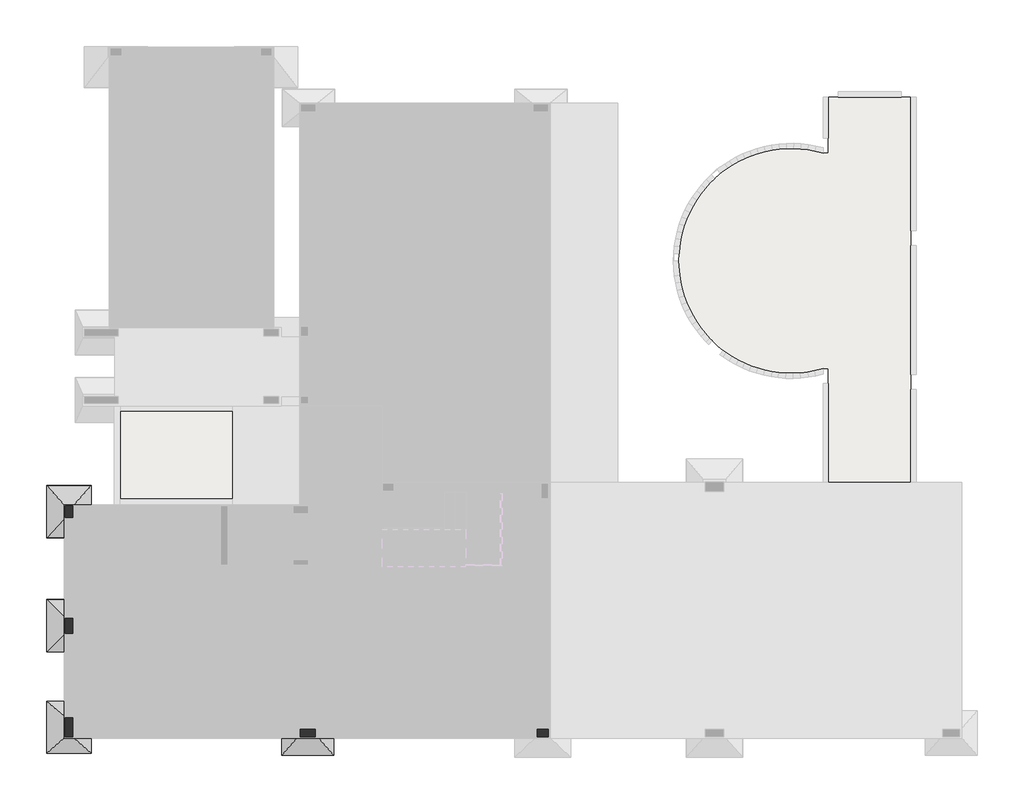
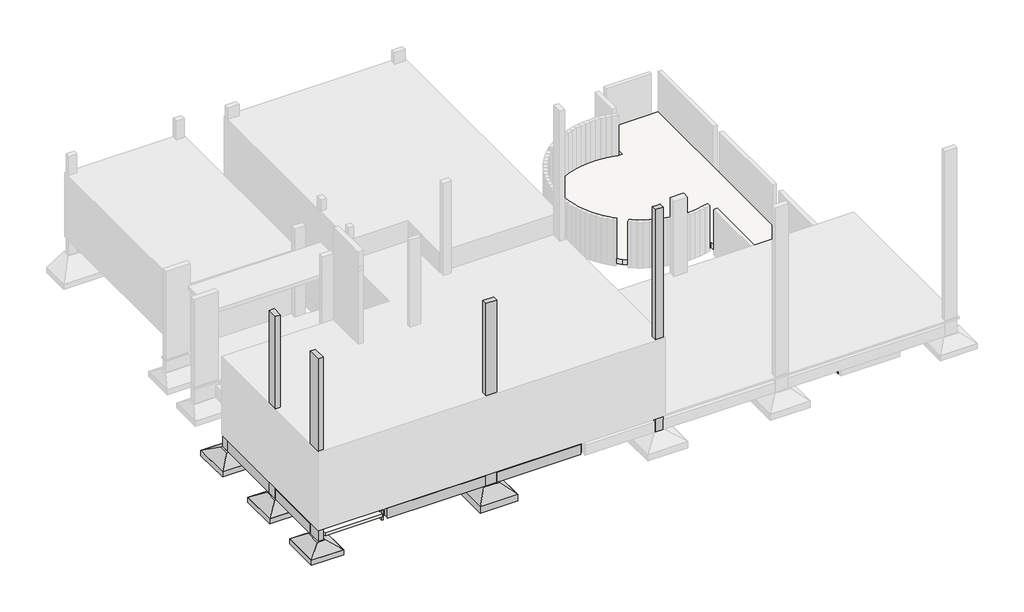
# One storey, part 1 of 4: 11 beams, 5 columns, 4 fasteners, 3 slabs.
"""IFC4 building model written with IfcOpenShell, lengths in millimetres."""

import ifcopenshell
import ifcopenshell.guid

model = None  # the IFC model being written
_history = None  # IfcOwnerHistory: only IFC2X3 demands one
_inside = {}  # id of a spatial element -> (the spatial element, [elements in it])
_under = {}  # id of a project, library or spatial element -> (it, [spatial elements below it])
_declared = {}  # id of a project -> (the project, [libraries it declares])
_typed = {}  # id of a type object -> (the type object, [elements of that type])
_made_of = {}  # id of a material, layer set ... -> (it, [elements and type objects made of it])


def new_model(schema):
    """Start an empty IFC model of exactly this schema.

    Asked for "IFC4X3", IfcOpenShell would pick the latest addendum, in which some entities
    have other attributes; the version numbers below select the first issue.
    IFC2X3 requires an IfcOwnerHistory on every rooted entity: one is made here for all.
    """
    global model, _history
    if schema == "IFC4X3":
        model = ifcopenshell.file(schema_version=(4, 3, 0, 0))
    else:
        model = ifcopenshell.file(schema=schema)
    _inside.clear()
    _under.clear()
    _declared.clear()
    _typed.clear()
    _made_of.clear()
    _history = None
    if model.schema == "IFC2X3":
        org = make("IfcOrganization", Name="unknown")
        user = make(
            "IfcPersonAndOrganization",
            ThePerson=make("IfcPerson", FamilyName="unknown"),
            TheOrganization=org,
        )
        app = make(
            "IfcApplication",
            ApplicationDeveloper=org,
            Version="unknown",
            ApplicationFullName="unknown",
            ApplicationIdentifier="unknown",
        )
        _history = make(
            "IfcOwnerHistory",
            OwningUser=user,
            OwningApplication=app,
            ChangeAction="ADDED",
            CreationDate=0,
        )
    return model


def make(cls, **values):
    """One entity of the class cls with the attributes given. An attribute that is None is left unset."""
    return model.create_entity(
        cls, **{name: value for name, value in values.items() if value is not None}
    )


def rooted(cls, **values):
    """An entity with a GlobalId (a new one), such as an element, a storey or a relation."""
    return make(cls, GlobalId=ifcopenshell.guid.new(), OwnerHistory=_history, **values)


def si_unit(unit_type, name, prefix=None):
    """IfcSIUnit, for example si_unit("LENGTHUNIT", "METRE", prefix="MILLI")."""
    return make("IfcSIUnit", UnitType=unit_type, Prefix=prefix, Name=name)


def assignment(units):
    """IfcUnitAssignment: the units of a project."""
    return None if units is None else make("IfcUnitAssignment", Units=units)


def point(xyz):
    """IfcCartesianPoint."""
    return None if xyz is None else make("IfcCartesianPoint", Coordinates=xyz)


def direction(xyz):
    """IfcDirection."""
    return None if xyz is None else make("IfcDirection", DirectionRatios=xyz)


def frame(location, z_axis=None, x_axis=None):
    """IfcAxis2Placement3D, a coordinate frame: its origin and axes. An axis left out is left unset."""
    return make(
        "IfcAxis2Placement3D",
        Location=point(location),
        Axis=direction(z_axis),
        RefDirection=direction(x_axis),
    )


def frame_2d(location, x_axis=None):
    """IfcAxis2Placement2D, a coordinate frame in the plane: its origin and x axis."""
    return make(
        "IfcAxis2Placement2D", Location=point(location), RefDirection=direction(x_axis)
    )


def origin():
    """The frame at (0, 0, 0) with its axes left unset."""
    return frame((0.0, 0.0, 0.0))


def place(relative_to, where):
    """IfcLocalPlacement: puts the frame where relative to a parent placement (None: the world)."""
    return make(
        "IfcLocalPlacement", PlacementRelTo=relative_to, RelativePlacement=where
    )


def context(
    kind, dimensions, precision=None, world=None, true_north=None, identifier=None
):
    """IfcGeometricRepresentationContext, for example the 3D "Model" context."""
    return make(
        "IfcGeometricRepresentationContext",
        ContextIdentifier=identifier,
        ContextType=kind,
        CoordinateSpaceDimension=dimensions,
        Precision=precision,
        WorldCoordinateSystem=world,
        TrueNorth=true_north,
    )


def project(units=None, contexts=None):
    """IfcProject with its units and contexts."""
    return rooted(
        "IfcProject",
        Name="project",
        RepresentationContexts=contexts,
        UnitsInContext=assignment(units),
    )


def spatial(cls, under=None, at=None, **own):
    """A site, building, storey or space (cls), placed at a placement, below another one or the project."""
    s = rooted(cls, ObjectPlacement=at, **own)
    if under is not None:
        _under.setdefault(under.id(), (under, []))[1].append(s)
    return s


def polyline(points):
    """IfcPolyline through the points."""
    return make("IfcPolyline", Points=[point(p) for p in points])


def circle_curve(where, radius):
    """IfcCircle in the frame where."""
    return make("IfcCircle", Position=where, Radius=radius)


def trimmed(basis, trim1, trim2, sense, master):
    """IfcTrimmedCurve: the piece of a basis curve between two trims."""
    return make(
        "IfcTrimmedCurve",
        BasisCurve=basis,
        Trim1=trim1,
        Trim2=trim2,
        SenseAgreement=sense,
        MasterRepresentation=master,
    )


def segment(curve, same_sense, transition):
    """IfcCompositeCurveSegment."""
    return make(
        "IfcCompositeCurveSegment",
        Transition=transition,
        SameSense=same_sense,
        ParentCurve=curve,
    )


def composite_curve(segments, self_intersect=None):
    """IfcCompositeCurve: segments joined end to end."""
    return make("IfcCompositeCurve", Segments=segments, SelfIntersect=self_intersect)


def outline(outer, holes=None, kind="AREA"):
    """IfcArbitraryClosedProfileDef: a profile drawn as a closed curve; with holes, ...WithVoids."""
    if holes is None:
        return make("IfcArbitraryClosedProfileDef", ProfileType=kind, OuterCurve=outer)
    return make(
        "IfcArbitraryProfileDefWithVoids",
        ProfileType=kind,
        OuterCurve=outer,
        InnerCurves=holes,
    )


def extrude(swept, where, along, depth):
    """IfcExtrudedAreaSolid: the profile swept, set in the frame where, extruded along a direction by depth."""
    return make(
        "IfcExtrudedAreaSolid",
        SweptArea=swept,
        Position=where,
        ExtrudedDirection=direction(along),
        Depth=depth,
    )


def faces_of(points, faces, orient=None, outer=None):
    """IfcFace entities. A face is a list of loops; a loop is a list of indices into points, from 0.

    orient and outer hold one flag for each loop. By default every Orientation is true, the
    first loop of a face is its IfcFaceOuterBound and the others are IfcFaceBound.
    """
    made = []
    for i, loops in enumerate(faces):
        bounds = []
        for j, loop in enumerate(loops):
            is_outer = j == 0 if outer is None else outer[i][j]
            bounds.append(
                make(
                    "IfcFaceOuterBound" if is_outer else "IfcFaceBound",
                    Bound=make("IfcPolyLoop", Polygon=[points[k] for k in loop]),
                    Orientation=True if orient is None else orient[i][j],
                )
            )
        made.append(make("IfcFace", Bounds=bounds))
    return made


def faceted_brep(points, faces, orient=None, outer=None, voids=None):
    """IfcFacetedBrep: a solid bounded by flat faces; with voids (closed shells), ...WithVoids."""
    shared = [point(p) for p in points]
    hull = make("IfcClosedShell", CfsFaces=faces_of(shared, faces, orient, outer))
    if voids is None:
        return make("IfcFacetedBrep", Outer=hull)
    return make(
        "IfcFacetedBrepWithVoids",
        Outer=hull,
        Voids=[
            make(cls, CfsFaces=faces_of(shared, fs, o, b)) for cls, fs, o, b in voids
        ],
    )


def shape(context_of_items, identifier, shape_type, items):
    """IfcShapeRepresentation: the items that make up one representation, for example the "Body"."""
    return make(
        "IfcShapeRepresentation",
        ContextOfItems=context_of_items,
        RepresentationIdentifier=identifier,
        RepresentationType=shape_type,
        Items=items,
    )


def source(mapping_origin, context_of_items, identifier, shape_type, items):
    """IfcRepresentationMap: a shape defined once, which mapped items show again and again."""
    return make(
        "IfcRepresentationMap",
        MappingOrigin=mapping_origin,
        MappedRepresentation=shape(context_of_items, identifier, shape_type, items),
    )


def transform(
    local_origin,
    x_axis=None,
    y_axis=None,
    z_axis=None,
    scale=None,
    scale2=None,
    scale3=None,
    uniform=True,
):
    """IfcCartesianTransformationOperator3D, or its non-uniform kind. x_axis, y_axis, z_axis: its Axis1, 2, 3."""
    if uniform:
        return make(
            "IfcCartesianTransformationOperator3D",
            Axis1=direction(x_axis),
            Axis2=direction(y_axis),
            LocalOrigin=point(local_origin),
            Scale=scale,
            Axis3=direction(z_axis),
        )
    return make(
        "IfcCartesianTransformationOperator3DnonUniform",
        Axis1=direction(x_axis),
        Axis2=direction(y_axis),
        LocalOrigin=point(local_origin),
        Scale=scale,
        Axis3=direction(z_axis),
        Scale2=scale2,
        Scale3=scale3,
    )


def mapped(mapping_source, mapping_target):
    """IfcMappedItem: shows the shape of a source again, moved by a transform."""
    return make(
        "IfcMappedItem", MappingSource=mapping_source, MappingTarget=mapping_target
    )


def made_of(thing, what):
    """Note that an element or type object is made of a material, layer set ...; save() writes the relation."""
    if what is not None:
        _made_of.setdefault(what.id(), (what, []))[1].append(thing)
    return thing


def element(
    cls,
    number,
    at=None,
    inside=None,
    cuts=None,
    type_object=None,
    material=None,
    context=None,
    identifier="Body",
    shape_type=None,
    held_by="IfcProductDefinitionShape",
    body=None,
    shapes=None,
    **own,
):
    """One element of the class cls, such as IfcWall. Its Tag is "e" and its number.

    at: its placement. inside: the storey or other place that contains it. cuts: it is an
    opening in that element (IfcRelVoidsElement). A single representation is given by context,
    identifier, shape_type and body (its items); several are given by shapes. held_by: the class
    of the entity that holds the representations. save() writes the other relations.
    """
    e = rooted(cls, Tag="e%d" % number, ObjectPlacement=at, **own)
    if body is not None:
        shapes = [shape(context, identifier, shape_type, body)]
    if shapes is not None:
        e.Representation = make(held_by, Representations=shapes)
    if inside is not None:
        _inside.setdefault(inside.id(), (inside, []))[1].append(e)
    if cuts is not None:
        rooted(
            "IfcRelVoidsElement", RelatingBuildingElement=cuts, RelatedOpeningElement=e
        )
    if type_object is not None:
        _typed.setdefault(type_object.id(), (type_object, []))[1].append(e)
    return made_of(e, material)


def aggregate(whole, parts):
    """IfcRelAggregates: a whole, such as a stair, and the parts it consists of."""
    return rooted("IfcRelAggregates", RelatingObject=whole, RelatedObjects=parts)


def save(model, path):
    """Write the relations noted so far, then the file.

    IfcRelAggregates (storeys below a building ...), IfcRelContainedInSpatialStructure (elements
    in a storey), IfcRelDefinesByType, IfcRelAssociatesMaterial and IfcRelDeclares: one each for
    every whole, place, type object, material and project.
    """
    for whole, parts in _under.values():
        aggregate(whole, parts)
    for where, things in _inside.values():
        rooted(
            "IfcRelContainedInSpatialStructure",
            RelatedElements=things,
            RelatingStructure=where,
        )
    for kind, things in _typed.values():
        rooted("IfcRelDefinesByType", RelatedObjects=things, RelatingType=kind)
    for what, things in _made_of.values():
        rooted("IfcRelAssociatesMaterial", RelatedObjects=things, RelatingMaterial=what)
    for by, libraries in _declared.values():
        rooted("IfcRelDeclares", RelatingContext=by, RelatedDefinitions=libraries)
    model.write(path)


def plane_surface(at):
    """IfcPlane: the flat surface through the origin of the frame at, square to its z axis."""
    return make("IfcPlane", Position=at)


def revolved_surface(curve, axis_point, axis_direction):
    """IfcSurfaceOfRevolution: the curve turned about the line through axis_point along axis_direction."""
    return make(
        "IfcSurfaceOfRevolution",
        SweptCurve=make("IfcArbitraryOpenProfileDef", ProfileType="CURVE", Curve=curve),
        AxisPosition=make("IfcAxis1Placement", Location=point(axis_point), Axis=direction(axis_direction)),
    )


def advanced_brep(points, edges, surfaces, faces):
    """IfcAdvancedBrep: a solid bounded by faces that lie on surfaces and meet in shared edges.

    An edge is (start, end): straight between two places in points (the first is 0);
    or (start, end, curve); or (start, end, curve, False) where it runs against its curve.
    A face is (place in surfaces, loops), or (place, loops, False) where it looks against
    its surface's normal. A loop lists edges by number (the first is 1), with a minus sign
    where the edge is run from its end to its start. The first loop is the outer one.
    """
    corners = [point(p) for p in points]
    vertices = [make("IfcVertexPoint", VertexGeometry=c) for c in corners]
    made = []
    for start, end, *more in edges:
        made.append(
            make(
                "IfcEdgeCurve",
                EdgeStart=vertices[start],
                EdgeEnd=vertices[end],
                EdgeGeometry=more[0] if more else make("IfcPolyline", Points=[corners[start], corners[end]]),
                SameSense=more[1] if len(more) > 1 else True,
            )
        )
    hull = []
    for where, loops, *sense in faces:
        bounds = []
        for j, loop in enumerate(loops):
            ring = [make("IfcOrientedEdge", EdgeElement=made[abs(k) - 1], Orientation=k > 0) for k in loop]
            bounds.append(
                make(
                    "IfcFaceOuterBound" if j == 0 else "IfcFaceBound",
                    Bound=make("IfcEdgeLoop", EdgeList=ring),
                    Orientation=True,
                )
            )
        hull.append(make("IfcAdvancedFace", Bounds=bounds, FaceSurface=surfaces[where], SameSense=sense[0] if sense else True))
    return make("IfcAdvancedBrep", Outer=make("IfcClosedShell", CfsFaces=hull))


def s15_bbe72304(model_context):
    return source(origin(), model_context, "Body", "SolidModel", [
        faceted_brep([(-55.0, 0.0, 0.0), (-345.0, 0.0, 0.0), (-345.0, -400.0, 0.0), (-55.0, -400.0, 0.0), (400.0, 500.0, -300.0), (400.0, -900.0, -300.0), (-800.0, -900.0, -300.0), (-800.0, 500.0, -300.0)], [[[0, 1, 2, 3]], [[4, 5, 6, 7]], [[4, 7, 1, 0]], [[7, 6, 2, 1]], [[6, 5, 3, 2]], [[5, 4, 0, 3]]]),
        extrude(outline(polyline([(400.0, 500.0), (400.0, -900.0), (-800.0, -900.0), (-800.0, 500.0), (400.0, 500.0)])), frame((0.0, 0.0, -500.0), z_axis=(0.0, 0.0, 1.0), x_axis=(1.0, 0.0, 0.0)), (0.0, 0.0, 1.0), 200.0),
    ])


def s19_c62a4a8b(model_context):
    return source(origin(), model_context, "Body", "SolidModel", [
        faceted_brep([(-55.0, 50.0, 0.0), (-345.0, 50.0, 0.0), (-345.0, -450.0, 0.0), (-55.0, -450.0, 0.0), (400.0, 500.0, -300.0), (400.0, -900.0, -300.0), (-800.0, -900.0, -300.0), (-800.0, 500.0, -300.0)], [[[0, 1, 2, 3]], [[4, 5, 6, 7]], [[4, 7, 1, 0]], [[7, 6, 2, 1]], [[6, 5, 3, 2]], [[5, 4, 0, 3]]]),
        extrude(outline(polyline([(400.0, 500.0), (400.0, -900.0), (-800.0, -900.0), (-800.0, 500.0), (400.0, 500.0)])), frame((0.0, 0.0, -500.0), z_axis=(0.0, 0.0, 1.0), x_axis=(1.0, 0.0, 0.0)), (0.0, 0.0, 1.0), 200.0),
    ])


def s20_c409a0c5(model_context):
    return source(origin(), model_context, "Body", "SolidModel", [
        faceted_brep([(-55.0, 100.0, 0.0), (-345.0, 100.0, 0.0), (-345.0, -500.0, 0.0), (-55.0, -500.0, 0.0), (400.0, 500.0, -300.0), (400.0, -900.0, -300.0), (-800.0, -900.0, -300.0), (-800.0, 500.0, -300.0)], [[[0, 1, 2, 3]], [[4, 5, 6, 7]], [[4, 7, 1, 0]], [[7, 6, 2, 1]], [[6, 5, 3, 2]], [[5, 4, 0, 3]]]),
        extrude(outline(polyline([(400.0, 500.0), (400.0, -900.0), (-800.0, -900.0), (-800.0, 500.0), (400.0, 500.0)])), frame((0.0, 0.0, -500.0), z_axis=(0.0, 0.0, 1.0), x_axis=(1.0, 0.0, 0.0)), (0.0, 0.0, 1.0), 200.0),
    ])


def s21_dbbb6426(model_context):
    return source(origin(), model_context, "Body", "SolidModel", [
        faceted_brep([(-55.0, 100.0, 0.0), (-345.0, 100.0, 0.0), (-345.0, -500.0, 0.0), (-55.0, -500.0, 0.0), (400.0, 500.0, -350.0), (400.0, -900.0, -350.0), (-800.0, -900.0, -350.0), (-800.0, 500.0, -350.0)], [[[0, 1, 2, 3]], [[4, 5, 6, 7]], [[4, 7, 1, 0]], [[7, 6, 2, 1]], [[6, 5, 3, 2]], [[5, 4, 0, 3]]]),
        extrude(outline(polyline([(400.0, 500.0), (400.0, -900.0), (-800.0, -900.0), (-800.0, 500.0), (400.0, 500.0)])), frame((0.0, 0.0, -600.0), z_axis=(0.0, 0.0, 1.0), x_axis=(1.0, 0.0, 0.0)), (0.0, 0.0, 1.0), 250.0),
    ])


model = new_model("IFC4")

# Units and contexts
model_context = context("Model", 3, world=origin())
ifc_project = project(units=[si_unit("LENGTHUNIT", "METRE", prefix="MILLI")], contexts=[model_context])

# Site, building, storey
site = spatial("IfcSite", under=ifc_project)
building = spatial("IfcBuilding", under=site)
storey = spatial("IfcBuildingStorey", under=building, Name="PAVIMENTO TÉRREO", Elevation=500.0)

# Beams
placement = place(None, origin())
element("IfcBeam", 1, ObjectType="TQS - Viga retangular : 14.0 x 40.0", at=placement, inside=storey, context=model_context, shape_type="SweptSolid", body=[
    extrude(outline(composite_curve([segment(trimmed(circle_curve(frame_2d((-5370.081307, -9633.3699847)), 125.0), [point((-5300.081307, -9529.8084088))], [point((-5440.081307, -9529.8084088))], True, "CARTESIAN"), True, "CONTINUOUS"), segment(polyline([(-5440.081307, -9529.8084088), (-5440.081307, -6553.3699847), (-5300.081307, -6553.3699847), (-5300.081307, -9529.8084088)]), True, "CONTINUOUS")], self_intersect=False)), frame((0.0, 0.0, 30.0), z_axis=(0.0, 0.0, 1.0), x_axis=(1.0, 0.0, 0.0)), (0.0, 0.0, 1.0), 400.0),
    extrude(outline(composite_curve([segment(trimmed(circle_curve(frame_2d((-5370.081307, -9633.3699847)), 125.0), [point((-5440.081307, -9736.9315606))], [point((-5300.081307, -9736.9315606))], True, "CARTESIAN"), True, "CONTINUOUS"), segment(polyline([(-5300.081307, -9736.9315606), (-5300.081307, -10953.5699847), (-5440.081307, -10953.5699847), (-5440.081307, -9736.9315606)]), True, "CONTINUOUS")], self_intersect=False)), frame((0.0, 0.0, 30.0), z_axis=(0.0, 0.0, 1.0), x_axis=(1.0, 0.0, 0.0)), (0.0, 0.0, 1.0), 400.0),
])
element("IfcBeam", 2, ObjectType="TQS - Viga retangular : 14.0 x 40.0", at=placement, inside=storey, context=model_context, shape_type="SweptSolid", body=[
    extrude(outline(composite_curve([segment(trimmed(circle_curve(frame_2d((-10471.281307, -6483.3699847)), 125.0), [point((-10574.8428829, -6413.3699847))], [point((-10596.281307, -6483.3699847))], True, "CARTESIAN"), True, "CONTINUOUS"), segment(trimmed(circle_curve(frame_2d((-10471.281307, -6483.3699847)), 125.0), [point((-10596.281307, -6483.3699847))], [point((-10574.8428829, -6553.3699847))], True, "CARTESIAN"), True, "CONTINUOUS"), segment(polyline([(-10574.8428829, -6553.3699847), (-12740.281307, -6553.3699847), (-12740.281307, -6413.3699847), (-10574.8428829, -6413.3699847)]), True, "CONTINUOUS")], self_intersect=False)), frame((0.0, 0.0, 30.0), z_axis=(0.0, 0.0, 1.0), x_axis=(1.0, 0.0, 0.0)), (0.0, 0.0, 1.0), 400.0),
])
element("IfcBeam", 3, ObjectType="TQS - Viga retangular : 14.0 x 40.0", at=placement, inside=storey, context=model_context, shape_type="SweptSolid", body=[
    extrude(outline(composite_curve([segment(polyline([(-8829.281307, -6413.3699847), (-8829.281307, -6553.3699847), (-10367.7197311, -6553.3699847)]), True, "CONTINUOUS"), segment(trimmed(circle_curve(frame_2d((-10471.281307, -6483.3699847)), 125.0), [point((-10367.7197311, -6553.3699847))], [point((-10346.281307, -6483.3699847))], True, "CARTESIAN"), True, "CONTINUOUS"), segment(trimmed(circle_curve(frame_2d((-10471.281307, -6483.3699847)), 125.0), [point((-10346.281307, -6483.3699847))], [point((-10367.7197311, -6413.3699847))], True, "CARTESIAN"), True, "CONTINUOUS"), segment(polyline([(-10367.7197311, -6413.3699847), (-8829.281307, -6413.3699847)]), True, "CONTINUOUS")], self_intersect=False)), frame((0.0, 0.0, 30.0), z_axis=(0.0, 0.0, 1.0), x_axis=(1.0, 0.0, 0.0)), (0.0, 0.0, 1.0), 400.0),
])
element("IfcBeam", 4, ObjectType="TQS - Viga retangular : 14.0 x 40.0", at=placement, inside=storey, context=model_context, shape_type="AdvancedBrep", body=[
    advanced_brep(
    [(-10541.281307, -6379.8084088, 430.0), (-10401.281307, -6379.8084088, 430.0), (-10401.281307, -5165.5699847, 430.0), (-10541.281307, -5165.5699847, 430.0), (-10401.281307, -6379.8084088, 30.0), (-10401.281307, -5165.5699847, 30.0), (-10541.281307, -6379.8084088, 30.0), (-10541.281307, -5165.5699847, 30.0)],
    [
        (0, 1, circle_curve(frame((-10471.281307, -6483.3699847, 430.0), z_axis=(0.0, 0.0, -1.0), x_axis=(1.0, 0.0, 0.0)), 125.0)),
        (1, 2),
        (2, 3),
        (3, 0),
        (1, 4),
        (4, 5),
        (5, 2),
        (4, 6, circle_curve(frame((-10471.281307, -6483.3699847, 30.0), z_axis=(0.0, 0.0, 1.0), x_axis=(1.0, 0.0, 0.0)), 125.0)),
        (6, 7),
        (7, 5),
        (6, 0),
        (3, 7),
    ],
    [
        plane_surface(frame((-10541.281307, -5178.2699847, 430.0), z_axis=(0.0, 0.0, 1.0), x_axis=(0.0, -1.0, 0.0))),
        plane_surface(frame((-10401.281307, -5178.2699847, 430.0), z_axis=(1.0, 0.0, 0.0), x_axis=(0.0, -1.0, 0.0))),
        plane_surface(frame((-10401.281307, -5178.2699847, 30.0), z_axis=(0.0, 0.0, -1.0), x_axis=(0.0, -1.0, 0.0))),
        plane_surface(frame((-10541.281307, -5178.2699847, 30.0), z_axis=(-1.0, 0.0, 0.0), x_axis=(0.0, -1.0, 0.0))),
        revolved_surface(polyline([(-10346.281307, -6483.3699847, 430.0), (-10346.281307, -6483.3699847, 30.0)]), (-10471.281307, -6483.3699847, -1500.0), (0.0, 0.0, 1.0)),
        plane_surface(frame((-6852.981307, -5165.5699847, 430.0), z_axis=(0.0, 1.0, 0.0), x_axis=(-1.0, 0.0, 0.0))),
    ],
    [
        (0, [[1, 2, 3, 4]]),
        (1, [[5, 6, 7, -2]]),
        (2, [[8, 9, 10, -6]]),
        (3, [[11, -4, 12, -9]]),
        (4, [[-1, -11, -8, -5]]),
        (5, [[-3, -7, -10, -12]]),
    ],
),
    advanced_brep(
    [(-10401.281307, -10923.9706268, 30.0), (-10401.281307, -10923.9706268, 430.0), (-10492.521691, -10953.5699847, 430.0), (-10492.521691, -10953.5699847, 30.0), (-10541.281307, -6586.9315606, 430.0), (-10401.281307, -6586.9315606, 430.0), (-10401.281307, -6586.9315606, 30.0), (-10541.281307, -6586.9315606, 30.0), (-10541.281307, -10744.5699847, 430.0), (-10541.281307, -10884.5699847, 430.0), (-10541.281307, -10953.5699847, 430.0), (-10541.281307, -10953.5699847, 30.0), (-10541.281307, -10884.5699847, 30.0), (-10541.281307, -10744.5699847, 30.0), (-10541.281307, -10953.5699847, 200.0), (-10541.281307, -10953.5699847, 320.0)],
    [
        (0, 1),
        (1, 2, circle_curve(frame((-10411.281307, -11048.5699847, 430.0), z_axis=(0.0, 0.0, 1.0), x_axis=(1.0, 0.0, 0.0)), 125.0)),
        (2, 3),
        (3, 0, circle_curve(frame((-10411.281307, -11048.5699847, 30.0), z_axis=(0.0, 0.0, -1.0), x_axis=(1.0, 0.0, 0.0)), 125.0)),
        (4, 5, circle_curve(frame((-10471.281307, -6483.3699847, 430.0), z_axis=(0.0, 0.0, 1.0), x_axis=(1.0, 0.0, 0.0)), 125.0)),
        (5, 6),
        (6, 7, circle_curve(frame((-10471.281307, -6483.3699847, 30.0), z_axis=(0.0, 0.0, -1.0), x_axis=(1.0, 0.0, 0.0)), 125.0)),
        (7, 4),
        (4, 8),
        (8, 9),
        (9, 10),
        (10, 2),
        (1, 5),
        (0, 6),
        (3, 11),
        (11, 12),
        (12, 13),
        (13, 7),
        (11, 14),
        (14, 15),
        (15, 10),
    ],
    [
        revolved_surface(polyline([(-10286.281307, -11048.5699847, 430.0), (-10286.281307, -11048.5699847, 30.0)]), (-10411.281307, -11048.5699847, -1500.0), (0.0, 0.0, 1.0)),
        revolved_surface(polyline([(-10346.281307, -6483.3699847, 430.0), (-10346.281307, -6483.3699847, 30.0)]), (-10471.281307, -6483.3699847, -1500.0), (0.0, 0.0, 1.0)),
        plane_surface(frame((-10541.281307, -5178.2699847, 430.0), z_axis=(0.0, 0.0, 1.0), x_axis=(0.0, -1.0, 0.0))),
        plane_surface(frame((-10401.281307, -5178.2699847, 430.0), z_axis=(1.0, 0.0, 0.0), x_axis=(0.0, -1.0, 0.0))),
        plane_surface(frame((-10401.281307, -5178.2699847, 30.0), z_axis=(0.0, 0.0, -1.0), x_axis=(0.0, -1.0, 0.0))),
        plane_surface(frame((-10541.281307, -5178.2699847, 30.0), z_axis=(-1.0, 0.0, 0.0), x_axis=(0.0, -1.0, 0.0))),
        plane_surface(frame((-3158.981307, -10953.5699847, 30.0), z_axis=(0.0, -1.0, 0.0), x_axis=(-1.0, 0.0, 0.0))),
    ],
    [
        (0, [[1, 2, 3, 4]]),
        (1, [[5, 6, 7, 8]]),
        (2, [[-5, 9, 10, 11, 12, -2, 13]]),
        (3, [[-1, 14, -6, -13]]),
        (4, [[-7, -14, -4, 15, 16, 17, 18]]),
        (5, [[-8, -18, -17, -16, 19, 20, 21, -11, -10, -9]]),
        (6, [[-3, -12, -21, -20, -19, -15]]),
    ],
),
])
element("IfcBeam", 5, ObjectType="TQS - Viga retangular : 14.0 x 40.0", at=placement, inside=storey, context=model_context, shape_type="SweptSolid", body=[
    extrude(outline(composite_curve([segment(trimmed(circle_curve(frame_2d((-3021.281307, -9633.3699847)), 125.0), [point((-3124.8428828, -9563.3699847))], [point((-3146.281307, -9633.3699847))], True, "CARTESIAN"), True, "CONTINUOUS"), segment(trimmed(circle_curve(frame_2d((-3021.281307, -9633.3699847)), 125.0), [point((-3146.281307, -9633.3699847))], [point((-3124.8428828, -9703.3699847))], True, "CARTESIAN"), True, "CONTINUOUS"), segment(polyline([(-3124.8428828, -9703.3699847), (-5266.5197311, -9703.3699847)]), True, "CONTINUOUS"), segment(trimmed(circle_curve(frame_2d((-5370.081307, -9633.3699847)), 125.0), [point((-5266.5197311, -9703.3699847))], [point((-5245.081307, -9633.3699847))], True, "CARTESIAN"), True, "CONTINUOUS"), segment(trimmed(circle_curve(frame_2d((-5370.081307, -9633.3699847)), 125.0), [point((-5245.081307, -9633.3699847))], [point((-5266.5197311, -9563.3699847))], True, "CARTESIAN"), True, "CONTINUOUS"), segment(polyline([(-5266.5197311, -9563.3699847), (-3124.8428828, -9563.3699847)]), True, "CONTINUOUS")], self_intersect=False)), frame((0.0, 0.0, 30.0), z_axis=(0.0, 0.0, 1.0), x_axis=(1.0, 0.0, 0.0)), (0.0, 0.0, 1.0), 400.0),
])
element("IfcBeam", 6, ObjectType="TQS - Viga retangular : 14.0 x 40.0", at=placement, inside=storey, context=model_context, shape_type="SweptSolid", body=[
    extrude(outline(composite_curve([segment(trimmed(circle_curve(frame_2d((-3021.281307, -11048.5699847)), 125.0), [point((-2951.281307, -10945.0084088))], [point((-3091.281307, -10945.0084088))], True, "CARTESIAN"), True, "CONTINUOUS"), segment(polyline([(-3091.281307, -10945.0084088), (-3091.281307, -9736.9315606)]), True, "CONTINUOUS"), segment(trimmed(circle_curve(frame_2d((-3021.281307, -9633.3699847)), 125.0), [point((-3091.281307, -9736.9315606))], [point((-2951.281307, -9736.9315606))], True, "CARTESIAN"), True, "CONTINUOUS"), segment(polyline([(-2951.281307, -9736.9315606), (-2951.281307, -10945.0084088)]), True, "CONTINUOUS")], self_intersect=False)), frame((0.0, 0.0, -60.0), z_axis=(0.0, 0.0, 1.0), x_axis=(1.0, 0.0, 0.0)), (0.0, 0.0, 1.0), 400.0),
])
element("IfcBeam", 7, ObjectType="TQS - Viga retangular : 14.0 x 40.0", at=placement, inside=storey, context=model_context, shape_type="SweptSolid", body=[
    extrude(outline(composite_curve([segment(trimmed(circle_curve(frame_2d((-3021.281307, -9633.3699847)), 125.0), [point((-2896.281307, -9633.3699847))], [point((-2917.7197311, -9563.3699847))], True, "CARTESIAN"), True, "CONTINUOUS"), segment(polyline([(-2917.7197311, -9563.3699847), (-202.281307, -9563.3699847), (-202.281307, -9703.3699847), (-2917.7197311, -9703.3699847)]), True, "CONTINUOUS"), segment(trimmed(circle_curve(frame_2d((-3021.281307, -9633.3699847)), 125.0), [point((-2917.7197311, -9703.3699847))], [point((-2896.281307, -9633.3699847))], True, "CARTESIAN"), True, "CONTINUOUS")], self_intersect=False)), frame((0.0, 0.0, -60.0), z_axis=(0.0, 0.0, 1.0), x_axis=(1.0, 0.0, 0.0)), (0.0, 0.0, 1.0), 400.0),
])
element("IfcBeam", 8, ObjectType="TQS - Viga retangular : 14.0 x 40.0", at=placement, inside=storey, context=model_context, shape_type="Brep", body=[
    faceted_brep([(-12690.2813069, -10744.5699847, 430.0), (-12690.2813069, -10744.5699847, 30.0), (-12690.2813069, -10884.5699847, 30.0), (-12690.2813069, -10884.5699847, 200.0), (-12690.2813069, -10884.5699847, 320.0), (-12690.2813069, -10884.5699847, 430.0), (-10541.281307, -10884.5699847, 430.0), (-10541.281307, -10744.5699847, 430.0), (-10541.281307, -10884.5699847, 30.0), (-10541.281307, -10884.5699847, 200.0), (-10541.281307, -10884.5699847, 320.0), (-10541.281307, -10744.5699847, 30.0)], [[[0, 1, 2, 3, 4, 5]], [[0, 5, 6, 7]], [[5, 4, 3, 2, 8, 9, 10, 6]], [[2, 1, 11, 8]], [[1, 0, 7, 11]], [[7, 6, 10, 9, 8, 11]]]),
])
element("IfcBeam", 9, ObjectType="TQS - Viga retangular : 19.0 x 40.0", at=placement, inside=storey, context=model_context, shape_type="Brep", body=[
    faceted_brep([(-12930.281307, -7975.5699847, 430.0), (-12740.281307, -7975.5699847, 430.0), (-12740.281307, -6553.3699847, 430.0), (-12740.281307, -6413.3699847, 430.0), (-12740.281307, -5275.5699847, 430.0), (-12930.281307, -5275.5699847, 430.0), (-12740.281307, -7975.5699847, 30.0), (-12740.281307, -6553.3699847, 30.0), (-12740.281307, -6413.3699847, 30.0), (-12740.281307, -5275.5699847, 30.0), (-12930.281307, -7975.5699847, 30.0), (-12930.281307, -5275.5699847, 30.0)], [[[0, 1, 2, 3, 4, 5]], [[1, 6, 7, 8, 9, 4, 3, 2]], [[6, 10, 11, 9, 8, 7]], [[10, 0, 5, 11]], [[1, 0, 10, 6]], [[5, 4, 9, 11]]]),
    faceted_brep([(-12930.281307, -8375.5699847, 430.0), (-12740.281307, -8375.5699847, 430.0), (-12740.281307, -8375.5699847, 30.0), (-12930.281307, -8375.5699847, 30.0), (-12930.281307, -10643.5699847, 430.0), (-12740.281307, -10643.5699847, 430.0), (-12740.281307, -10643.5699847, 30.0), (-12930.281307, -10643.5699847, 30.0)], [[[0, 1, 2, 3]], [[1, 0, 4, 5]], [[2, 1, 5, 6]], [[3, 2, 6, 7]], [[0, 3, 7, 4]], [[5, 4, 7, 6]]]),
])
element("IfcBeam", 10, ObjectType="TQS - Viga retangular : 19.0 x 40.0", at=placement, inside=storey, context=model_context, shape_type="AdvancedBrep", body=[
    advanced_brep(
    [(-6249.181307, -10953.5699847, 430.0), (-6249.181307, -11143.5699847, 430.0), (-3102.521691, -11143.5699847, 430.0), (-3146.281307, -11048.5699847, 430.0), (-3102.521691, -10953.5699847, 430.0), (-5300.081307, -10953.5699847, 430.0), (-5440.081307, -10953.5699847, 430.0), (-6249.181307, -11143.5699847, 30.0), (-3102.521691, -11143.5699847, 30.0), (-6249.181307, -10953.5699847, 30.0), (-5440.081307, -10953.5699847, 30.0), (-5300.081307, -10953.5699847, 30.0), (-3102.521691, -10953.5699847, 30.0), (-3146.281307, -11048.5699847, 30.0)],
    [
        (0, 1),
        (1, 2),
        (2, 3, circle_curve(frame((-3021.281307, -11048.5699847, 430.0), z_axis=(0.0, 0.0, -1.0), x_axis=(1.0, 0.0, 0.0)), 125.0)),
        (3, 4, circle_curve(frame((-3021.281307, -11048.5699847, 430.0), z_axis=(0.0, 0.0, -1.0), x_axis=(1.0, 0.0, 0.0)), 125.0)),
        (4, 5),
        (5, 6),
        (6, 0),
        (1, 7),
        (7, 8),
        (8, 2),
        (7, 9),
        (9, 10),
        (10, 11),
        (11, 12),
        (12, 13, circle_curve(frame((-3021.281307, -11048.5699847, 30.0), z_axis=(0.0, 0.0, 1.0), x_axis=(1.0, 0.0, 0.0)), 125.0)),
        (13, 8, circle_curve(frame((-3021.281307, -11048.5699847, 30.0), z_axis=(0.0, 0.0, 1.0), x_axis=(1.0, 0.0, 0.0)), 125.0)),
        (9, 0),
        (4, 12),
        (3, 13),
    ],
    [
        plane_surface(frame((-3158.981307, -10953.5699847, 430.0), z_axis=(0.0, 0.0, 1.0), x_axis=(-1.0, 0.0, 0.0))),
        plane_surface(frame((-3158.981307, -11143.5699847, 430.0), z_axis=(0.0, -1.0, 0.0), x_axis=(-1.0, 0.0, 0.0))),
        plane_surface(frame((-3158.981307, -11143.5699847, 30.0), z_axis=(0.0, 0.0, -1.0), x_axis=(-1.0, 0.0, 0.0))),
        plane_surface(frame((-3158.981307, -10953.5699847, 30.0), z_axis=(0.0, 1.0, 0.0), x_axis=(-1.0, 0.0, 0.0))),
        plane_surface(frame((-6249.181307, -11143.5699847, 7250.0), z_axis=(-1.0, 0.0, 0.0), x_axis=(0.0, 0.0, -1.0))),
        revolved_surface(polyline([(-2896.281307, -11048.5699847, 430.0), (-2896.281307, -11048.5699847, 30.0)]), (-3021.281307, -11048.5699847, -1500.0), (0.0, 0.0, 1.0)),
    ],
    [
        (0, [[1, 2, 3, 4, 5, 6, 7]]),
        (1, [[8, 9, 10, -2]]),
        (2, [[11, 12, 13, 14, 15, 16, -9]]),
        (3, [[17, -7, -6, -5, 18, -14, -13, -12]]),
        (4, [[-1, -17, -11, -8]]),
        (5, [[19, -15, -18, -4]]),
        (5, [[-19, -3, -10, -16]]),
    ],
),
    advanced_brep(
    [(-6649.181307, -10953.5699847, 430.0), (-6649.181307, -11143.5699847, 430.0), (-6649.181307, -11143.5699847, 30.0), (-6649.181307, -10953.5699847, 30.0), (-10330.0409229, -10953.5699847, 430.0), (-10286.281307, -11048.5699847, 430.0), (-10330.0409229, -11143.5699847, 430.0), (-10330.0409229, -11143.5699847, 30.0), (-10286.281307, -11048.5699847, 30.0), (-10330.0409229, -10953.5699847, 30.0)],
    [
        (0, 1),
        (1, 2),
        (2, 3),
        (3, 0),
        (0, 4),
        (4, 5, circle_curve(frame((-10411.281307, -11048.5699847, 430.0), z_axis=(0.0, 0.0, -1.0), x_axis=(1.0, 0.0, 0.0)), 125.0)),
        (5, 6, circle_curve(frame((-10411.281307, -11048.5699847, 430.0), z_axis=(0.0, 0.0, -1.0), x_axis=(1.0, 0.0, 0.0)), 125.0)),
        (6, 1),
        (6, 7),
        (7, 2),
        (7, 8, circle_curve(frame((-10411.281307, -11048.5699847, 30.0), z_axis=(0.0, 0.0, 1.0), x_axis=(1.0, 0.0, 0.0)), 125.0)),
        (8, 9, circle_curve(frame((-10411.281307, -11048.5699847, 30.0), z_axis=(0.0, 0.0, 1.0), x_axis=(1.0, 0.0, 0.0)), 125.0)),
        (9, 3),
        (9, 4),
        (8, 5),
    ],
    [
        plane_surface(frame((-6649.181307, -10953.5699847, 7250.0), z_axis=(1.0, 0.0, 0.0), x_axis=(0.0, 0.0, -1.0))),
        plane_surface(frame((-3158.981307, -10953.5699847, 430.0), z_axis=(0.0, 0.0, 1.0), x_axis=(-1.0, 0.0, 0.0))),
        plane_surface(frame((-3158.981307, -11143.5699847, 430.0), z_axis=(0.0, -1.0, 0.0), x_axis=(-1.0, 0.0, 0.0))),
        plane_surface(frame((-3158.981307, -11143.5699847, 30.0), z_axis=(0.0, 0.0, -1.0), x_axis=(-1.0, 0.0, 0.0))),
        plane_surface(frame((-3158.981307, -10953.5699847, 30.0), z_axis=(0.0, 1.0, 0.0), x_axis=(-1.0, 0.0, 0.0))),
        revolved_surface(polyline([(-10286.281307, -11048.5699847, 430.0), (-10286.281307, -11048.5699847, 30.0)]), (-10411.281307, -11048.5699847, -1500.0), (0.0, 0.0, 1.0)),
    ],
    [
        (0, [[1, 2, 3, 4]]),
        (1, [[-1, 5, 6, 7, 8]]),
        (2, [[-2, -8, 9, 10]]),
        (3, [[-3, -10, 11, 12, 13]]),
        (4, [[-4, -13, 14, -5]]),
        (5, [[15, -6, -14, -12]]),
        (5, [[-15, -11, -9, -7]]),
    ],
),
    advanced_brep(
    [(-10536.281307, -11048.5699847, 30.0), (-10536.281307, -11048.5699847, 430.0), (-10492.521691, -11143.5699847, 430.0), (-10492.521691, -11143.5699847, 30.0), (-10541.281307, -11143.5699847, 430.0), (-10541.281307, -10953.5699847, 430.0), (-10541.281307, -10953.5699847, 30.0), (-10541.281307, -11143.5699847, 30.0), (-10492.521691, -10953.5699847, 430.0), (-10492.521691, -10953.5699847, 30.0)],
    [
        (0, 1),
        (1, 2, circle_curve(frame((-10411.281307, -11048.5699847, 430.0), z_axis=(0.0, 0.0, 1.0), x_axis=(1.0, 0.0, 0.0)), 125.0)),
        (2, 3),
        (3, 0, circle_curve(frame((-10411.281307, -11048.5699847, 30.0), z_axis=(0.0, 0.0, -1.0), x_axis=(1.0, 0.0, 0.0)), 125.0)),
        (4, 5),
        (5, 6),
        (6, 7),
        (7, 4),
        (4, 2),
        (1, 8, circle_curve(frame((-10411.281307, -11048.5699847, 430.0), z_axis=(0.0, 0.0, -1.0), x_axis=(1.0, 0.0, 0.0)), 125.0)),
        (8, 5),
        (7, 3),
        (6, 9),
        (9, 0, circle_curve(frame((-10411.281307, -11048.5699847, 30.0), z_axis=(0.0, 0.0, 1.0), x_axis=(1.0, 0.0, 0.0)), 125.0)),
        (8, 9),
    ],
    [
        revolved_surface(polyline([(-10286.281307, -11048.5699847, 430.0), (-10286.281307, -11048.5699847, 30.0)]), (-10411.281307, -11048.5699847, -1500.0), (0.0, 0.0, 1.0)),
        plane_surface(frame((-10541.281307, -11167.4990682, 430.0), z_axis=(-1.0, 0.0, 0.0), x_axis=(0.0, 1.0, 0.0))),
        plane_surface(frame((-3158.981307, -10953.5699847, 430.0), z_axis=(0.0, 0.0, 1.0), x_axis=(-1.0, 0.0, 0.0))),
        plane_surface(frame((-3158.981307, -11143.5699847, 430.0), z_axis=(0.0, -1.0, 0.0), x_axis=(-1.0, 0.0, 0.0))),
        plane_surface(frame((-3158.981307, -11143.5699847, 30.0), z_axis=(0.0, 0.0, -1.0), x_axis=(-1.0, 0.0, 0.0))),
        plane_surface(frame((-3158.981307, -10953.5699847, 30.0), z_axis=(0.0, 1.0, 0.0), x_axis=(-1.0, 0.0, 0.0))),
    ],
    [
        (0, [[1, 2, 3, 4]]),
        (1, [[5, 6, 7, 8]]),
        (2, [[-5, 9, -2, 10, 11]]),
        (3, [[-8, 12, -3, -9]]),
        (4, [[-7, 13, 14, -4, -12]]),
        (5, [[-6, -11, 15, -13]]),
        (0, [[-1, -14, -15, -10]]),
    ],
),
])
element("IfcBeam", 11, ObjectType="TQS - Viga retangular : 19.0 x 55.0", at=placement, inside=storey, context=model_context, shape_type="Brep", body=[
    faceted_brep([(-6840.281307, -5165.5699847, 430.0), (-6840.281307, -4975.5699847, 430.0), (-8589.281307, -4975.5699847, 430.0), (-8589.281307, -5165.5699847, 430.0), (-12740.281307, -5165.5699847, 30.0), (-12930.281307, -5165.5699847, 30.0), (-12930.281307, -5165.5699847, -120.0), (-6440.281307, -5165.5699847, -120.0), (-6440.281307, -5165.5699847, 30.0), (-6840.281307, -5165.5699847, 30.0), (-8589.281307, -5165.5699847, -100.0), (-8779.281307, -5165.5699847, -100.0), (-8779.281307, -5165.5699847, 430.0), (-10401.281307, -5165.5699847, 430.0), (-10541.281307, -5165.5699847, 430.0), (-12740.281307, -5165.5699847, 430.0), (-12930.281307, -4975.5699847, -120.0), (-6440.281307, -4975.5699847, -120.0), (-12930.281307, -4975.5699847, 30.0), (-12740.281307, -4975.5699847, 30.0), (-12740.281307, -4975.5699847, 430.0), (-8779.281307, -4975.5699847, 430.0), (-8779.281307, -4975.5699847, -100.0), (-8589.281307, -4975.5699847, -100.0), (-6840.281307, -4975.5699847, 30.0), (-6440.281307, -4975.5699847, 30.0)], [[[0, 1, 2, 3]], [[4, 5, 6, 7, 8, 9, 0, 3, 10, 11, 12, 13, 14, 15]], [[6, 16, 17, 7]], [[18, 19, 20, 21, 22, 23, 2, 1, 24, 25, 17, 16]], [[4, 19, 18, 5]], [[19, 4, 15, 20]], [[24, 9, 8, 25]], [[9, 24, 1, 0]], [[10, 23, 22, 11]], [[11, 22, 21, 12]], [[23, 10, 3, 2]], [[20, 15, 14, 13, 12, 21]], [[16, 6, 5, 18]], [[7, 17, 25, 8]]]),
])

# Columns
element("IfcColumn", 12, ObjectType="TQS - Pilar retangular : 19.0 x 30.0", at=placement, inside=storey, context=model_context, shape_type="Brep", body=[
    faceted_brep([(-312.281307, -10953.5699847, -60.0), (-202.281307, -10953.5699847, -60.0), (-12.281307, -10953.5699847, -60.0), (-12.281307, -11143.5699847, -60.0), (-312.281307, -11143.5699847, -60.0), (-312.281307, -10953.5699847, 8750.0), (-152.281307, -10953.5699847, 8750.0), (-12.281307, -10953.5699847, 8750.0), (-12.281307, -10953.5699847, 8300.0), (-12.281307, -10953.5699847, 7250.0), (-12.281307, -10953.5699847, 7050.0), (-12.281307, -10953.5699847, 6450.0), (-12.281307, -10953.5699847, 3530.0), (-12.281307, -10953.5699847, 3080.0), (-12.281307, -10953.5699847, 3030.0), (-12.281307, -10953.5699847, 340.0), (-312.281307, -10953.5699847, 340.0), (-312.281307, -10953.5699847, 3030.0), (-312.281307, -10953.5699847, 3530.0), (-312.281307, -10953.5699847, 6450.0), (-312.281307, -10953.5699847, 7250.0), (-12.281307, -11003.5699847, 8750.0), (-12.281307, -11143.5699847, 8750.0), (-12.281307, -11143.5699847, 8300.0), (-12.281307, -11143.5699847, 7250.0), (-12.281307, -11143.5699847, 6450.0), (-12.281307, -11143.5699847, 3530.0), (-12.281307, -11143.5699847, 3030.0), (-12.281307, -11143.5699847, 340.0), (-312.281307, -11143.5699847, 8750.0), (-312.281307, -11143.5699847, 7250.0), (-312.281307, -11143.5699847, 6450.0), (-312.281307, -11143.5699847, 3530.0), (-312.281307, -11143.5699847, 3030.0), (-312.281307, -11143.5699847, 340.0)], [[[0, 1, 2, 3, 4]], [[5, 6, 7, 8, 9, 10, 11, 12, 13, 14, 15, 2, 1, 0, 16, 17, 18, 19, 20]], [[7, 21, 22, 23, 24, 25, 26, 27, 28, 3, 2, 15, 14, 13, 12, 11, 10, 9, 8]], [[22, 29, 30, 31, 32, 33, 34, 4, 3, 28, 27, 26, 25, 24, 23]], [[29, 5, 20, 19, 18, 17, 16, 0, 4, 34, 33, 32, 31, 30]], [[5, 29, 22, 21, 7, 6]]]),
])
element("IfcColumn", 13, ObjectType="TQS - Pilar retangular : 19.0 x 30.0", at=placement, inside=storey, context=model_context, shape_type="Brep", body=[
    faceted_brep([(-12740.281307, -4975.5699847, 30.0), (-12740.281307, -5165.5699847, 30.0), (-12740.281307, -5275.5699847, 30.0), (-12930.281307, -5275.5699847, 30.0), (-12930.281307, -5165.5699847, 30.0), (-12930.281307, -4975.5699847, 30.0), (-12740.281307, -4975.5699847, 3530.0), (-12740.281307, -5165.5699937, 3530.0), (-12740.281307, -5275.5699847, 3530.0), (-12740.281307, -5275.5699847, 3030.0), (-12740.281307, -5275.5699847, 430.0), (-12740.281307, -4975.5699847, 430.0), (-12930.281307, -5275.5699847, 3530.0), (-12930.281307, -5275.5699847, 3030.0), (-12930.281307, -5275.5699847, 430.0), (-12930.281307, -4975.5699847, 3530.0)], [[[0, 1, 2, 3, 4, 5]], [[6, 7, 8, 9, 10, 2, 1, 0, 11]], [[8, 12, 13, 14, 3, 2, 10, 9]], [[12, 15, 5, 4, 3, 14, 13]], [[15, 6, 11, 0, 5]], [[6, 15, 12, 8, 7]]]),
])
element("IfcColumn", 14, ObjectType="TQS - Pilar retangular : 19.0 x 40.0", at=placement, inside=storey, context=model_context, shape_type="Brep", body=[
    faceted_brep([(-12740.2813069, -7975.5699847, 30.0), (-12740.2813069, -8375.5699847, 30.0), (-12930.2813069, -8375.5699847, 30.0), (-12930.2813069, -7975.5699847, 30.0), (-12740.2813069, -7975.5699847, 7260.5), (-12740.2813069, -8375.5699847, 7260.5), (-12740.2813069, -8375.5699847, 6360.5), (-12740.2813069, -8375.5699847, 6350.0), (-12740.2813069, -8375.5699847, 5850.0), (-12740.2813069, -8375.5699847, 4480.0), (-12740.2813069, -8375.5699847, 4030.0), (-12740.2813069, -8375.5699847, 3530.0), (-12740.2813069, -8375.5699847, 3030.0), (-12740.2813069, -8375.5699847, 430.0), (-12740.2813069, -7975.5699847, 430.0), (-12740.2813069, -7975.5699847, 3030.0), (-12740.2813069, -7975.5699847, 3530.0), (-12740.2813069, -7975.5699847, 4030.0), (-12740.2813069, -7975.5699847, 4480.0), (-12740.2813069, -7975.5699847, 5850.0), (-12740.2813069, -7975.5699847, 6350.0), (-12740.2813069, -7975.5699847, 6360.5), (-12930.2813069, -8375.5699847, 7260.5), (-12930.2813069, -8375.5699847, 6360.5), (-12930.2813069, -8375.5699847, 6350.0), (-12930.2813069, -8375.5699847, 5850.0), (-12930.2813069, -8375.5699847, 4480.0), (-12930.2813069, -8375.5699847, 4030.0), (-12930.2813069, -8375.5699847, 3530.0), (-12930.2813069, -8375.5699847, 3030.0), (-12930.2813069, -8375.5699847, 430.0), (-12930.2813069, -7975.5699847, 7260.5), (-12930.2813069, -7975.5699847, 6360.5), (-12930.2813069, -7975.5699847, 6350.0), (-12930.2813069, -7975.5699847, 5850.0), (-12930.2813069, -7975.5699847, 4480.0), (-12930.2813069, -7975.5699847, 4030.0), (-12930.2813069, -7975.5699847, 3530.0), (-12930.2813069, -7975.5699847, 3030.0), (-12930.2813069, -7975.5699847, 430.0)], [[[0, 1, 2, 3]], [[4, 5, 6, 7, 8, 9, 10, 11, 12, 13, 1, 0, 14, 15, 16, 17, 18, 19, 20, 21]], [[5, 22, 23, 24, 25, 26, 27, 28, 29, 30, 2, 1, 13, 12, 11, 10, 9, 8, 7, 6]], [[22, 31, 32, 33, 34, 35, 36, 37, 38, 39, 3, 2, 30, 29, 28, 27, 26, 25, 24, 23]], [[31, 4, 21, 20, 19, 18, 17, 16, 15, 14, 0, 3, 39, 38, 37, 36, 35, 34, 33, 32]], [[4, 31, 22, 5]]]),
])
element("IfcColumn", 15, ObjectType="TQS - Pilar retangular : 19.0 x 40.0", at=placement, inside=storey, context=model_context, shape_type="Brep", body=[
    faceted_brep([(-6249.181307, -11143.5699847, 30.0), (-6649.181307, -11143.5699847, 30.0), (-6649.181307, -10953.5699847, 30.0), (-6249.181307, -10953.5699847, 30.0), (-6249.181307, -11143.5699847, 7250.0), (-6649.181307, -11143.5699847, 7250.0), (-6649.181307, -11143.5699847, 6450.0), (-6649.181307, -11143.5699847, 3530.0), (-6649.181307, -11143.5699847, 3030.0), (-6649.181307, -11143.5699847, 430.0), (-6249.181307, -11143.5699847, 430.0), (-6249.181307, -11143.5699847, 3030.0), (-6249.181307, -11143.5699847, 3530.0), (-6249.181307, -11143.5699847, 6450.0), (-6649.181307, -10953.5699847, 7250.0), (-6649.181307, -10953.5699847, 6450.0), (-6649.181307, -10953.5699847, 3530.0), (-6649.181307, -10953.5699847, 3030.0), (-6649.181307, -10953.5699847, 430.0), (-6249.181307, -10953.5699847, 7250.0), (-6249.181307, -10953.5699847, 6450.0), (-6249.181307, -10953.5699847, 3530.0), (-6249.181307, -10953.5699847, 3030.0), (-6249.181307, -10953.5699847, 430.0)], [[[0, 1, 2, 3]], [[4, 5, 6, 7, 8, 9, 1, 0, 10, 11, 12, 13]], [[5, 14, 15, 16, 17, 18, 2, 1, 9, 8, 7, 6]], [[14, 19, 20, 21, 22, 23, 3, 2, 18, 17, 16, 15]], [[19, 4, 13, 12, 11, 10, 0, 3, 23, 22, 21, 20]], [[4, 19, 14, 5]]]),
])
element("IfcColumn", 16, ObjectType="TQS - Pilar retangular : 19.0 x 50.0", at=placement, inside=storey, context=model_context, shape_type="Brep", body=[
    faceted_brep([(-12740.2813069, -10643.5699847, 30.0), (-12740.2813069, -11143.5699847, 30.0), (-12930.2813069, -11143.5699847, 30.0), (-12930.2813069, -10643.5699847, 30.0), (-12740.2813069, -10643.5699847, 7260.5), (-12740.2813069, -11143.5699847, 7260.5), (-12740.2813069, -11143.5699847, 7250.0), (-12740.2813069, -11143.5699847, 6450.0), (-12740.2813069, -11143.5699847, 3530.0), (-12740.2813069, -11143.5699847, 3030.0), (-12740.2813069, -10643.5699847, 430.0), (-12740.2813069, -10643.5699847, 3030.0), (-12740.2813069, -10643.5699847, 3530.0), (-12740.2813069, -10643.5699847, 4030.0), (-12740.2813069, -10643.5699847, 4480.0), (-12740.2813069, -10643.5699847, 5850.0), (-12740.2813069, -10643.5699847, 6350.0), (-12740.2813069, -10643.5699847, 6360.5), (-12740.2813069, -10643.5699847, 7057.5873816), (-12740.2813069, -10643.5699847, 7062.9382478), (-12930.2813069, -11143.5699847, 7260.5), (-12930.2813069, -10643.5699847, 7260.5), (-12930.2813069, -10643.5699847, 6360.5), (-12930.2813069, -10643.5699847, 6350.0), (-12930.2813069, -10643.5699847, 5850.0), (-12930.2813069, -10643.5699847, 4480.0), (-12930.2813069, -10643.5699847, 4030.0), (-12930.2813069, -10643.5699847, 3530.0), (-12930.2813069, -10643.5699847, 3030.0), (-12930.2813069, -10643.5699847, 430.0)], [[[0, 1, 2, 3]], [[4, 5, 6, 7, 8, 9, 1, 0, 10, 11, 12, 13, 14, 15, 16, 17, 18, 19]], [[5, 20, 2, 1, 9, 8, 7, 6]], [[20, 21, 22, 23, 24, 25, 26, 27, 28, 29, 3, 2]], [[21, 4, 19, 18, 17, 16, 15, 14, 13, 12, 11, 10, 0, 3, 29, 28, 27, 26, 25, 24, 23, 22]], [[4, 21, 20, 5]]]),
])

# Fasteners
s15_shape = s15_bbe72304(model_context)
element("IfcFastener", 17, ObjectType="TQS - Sapata : S15", at=placement, inside=storey, context=model_context, shape_type="MappedRepresentation", body=[
    mapped(s15_shape, transform((-12635.281307, -4925.5699847, 30.0), x_axis=(1.0, 0.0, 0.0), y_axis=(0.0, 1.0, 0.0), z_axis=(0.0, 0.0, 1.0))),
])
s19_shape = s19_c62a4a8b(model_context)
element("IfcFastener", 18, ObjectType="TQS - Sapata : S19", at=placement, inside=storey, context=model_context, shape_type="MappedRepresentation", body=[
    mapped(s19_shape, transform((-12635.2813069, -7975.5699847, 30.0), x_axis=(1.0, 0.0, 0.0), y_axis=(0.0, 1.0, 0.0), z_axis=(0.0, 0.0, 1.0))),
])
s20_shape = s20_c409a0c5(model_context)
element("IfcFastener", 19, ObjectType="TQS - Sapata : S20", at=placement, inside=storey, context=model_context, shape_type="MappedRepresentation", body=[
    mapped(s20_shape, transform((-13035.2813069, -11093.5699847, 30.0), x_axis=(-1.0, 0.0, 0.0), y_axis=(0.0, -1.0, 0.0), z_axis=(0.0, 0.0, 1.0))),
])
s21_shape = s21_dbbb6426(model_context)
element("IfcFastener", 20, ObjectType="TQS - Sapata : S21", at=placement, inside=storey, context=model_context, shape_type="MappedRepresentation", body=[
    mapped(s21_shape, transform((-6649.181307, -10848.5699847, 30.0), x_axis=(0.0, 1.0, 0.0), y_axis=(-1.0, 0.0, 0.0), z_axis=(0.0, 0.0, 1.0))),
])

# Slabs
element("IfcSlab", 21, ObjectType="TQS h=12", at=placement, inside=storey, context=model_context, shape_type="SweptSolid", body=[
    extrude(outline(polyline([(-11470.281307, -4784.5699847), (-11470.281307, -2435.5749263), (-7728.281307, -2435.1126228), (-7728.281307, -2552.0699847), (-7672.281307, -2552.0699847), (-7672.281307, -4784.5699847), (-11470.281307, -4784.5699847)])), frame((0.0, 0.0, -120.0), z_axis=(0.0, 0.0, 1.0), x_axis=(1.0, 0.0, 0.0)), (0.0, 0.0, 1.0), 120.0),
])
element("IfcSlab", 22, ObjectType="TQS h=12", at=placement, inside=storey, context=model_context, shape_type="SweptSolid", body=[
    extrude(outline(polyline([(-12690.2813069, -10884.5699847), (-10541.281307, -10884.5699847), (-10541.281307, -11185.5699847), (-12690.2813069, -11185.5699847), (-12690.2813069, -10884.5699847)])), frame((0.0, 0.0, 200.0), z_axis=(0.0, 0.0, 1.0), x_axis=(1.0, 0.0, 0.0)), (0.0, 0.0, 1.0), 120.0),
])
element("IfcSlab", 23, ObjectType="TQS h=20", at=placement, inside=storey, context=model_context, shape_type="Brep", body=[
    faceted_brep([(7474.7218272, 4470.7003679, -1450.0), (7474.7218272, 4870.7003679, -1450.0), (7474.7218272, 5969.4300153, -1450.0), (7734.718693, 5969.4300153, -1450.0), (9422.718693, 5969.4300153, -1450.0), (9682.718693, 5969.4300153, -1450.0), (9682.718693, 2394.0144504, -1450.0), (9682.718693, 1994.0144504, -1450.0), (9682.718693, -1451.4011146, -1450.0), (9682.718693, -1851.4011146, -1450.0), (9682.718693, -5230.1494451, -1450.0), (9682.718693, -5630.1494451, -1450.0), (9682.718693, -9279.5699847, -1450.0), (9682.718693, -9539.5699847, -1450.0), (7474.718693, -9539.5699847, -1450.0), (7474.718693, -9279.5699847, -1450.0), (7474.718693, -5630.1494451, -1450.0), (7474.718693, -5230.1494451, -1450.0), (7474.718693, -1696.0936198, -1450.0), (7474.718693, -1296.0936198, -1450.0), (7334.718693, -1296.0936198, -1450.0), (7106.1277936, -1352.3610531, -1450.0), (6917.7849868, -1386.2922761, -1450.0), (6727.7008432, -1408.1801126, -1450.0), (6536.6098693, -1417.942206, -1450.0), (6345.2847953, -1415.5390805, -1450.0), (6154.4732894, -1400.978469, -1450.0), (5966.1413215, -1374.5554297, -1450.0), (5778.7697179, -1335.9166014, -1450.0), (5594.2076289, -1285.4399321, -1450.0), (5413.6522985, -1223.4807754, -1450.0), (5236.9847165, -1149.9982825, -1450.0), (5065.344906, -1065.4356735, -1450.0), (4899.4264221, -970.1346281, -1450.0), (4740.8701617, -865.1228032, -1450.0), (4665.976342, -808.0652799, -1450.0), (4515.316429, -686.0238096, -1450.0), (4362.9503182, -544.9436994, -1450.0), (4307.4254093, -490.9002096, -1450.0), (4179.8070625, -348.7027306, -1450.0), (4061.9329165, -199.2498808, -1450.0), (3953.2296156, -41.7867013, -1450.0), (3854.7542482, 122.2671329, -1450.0), (3766.9048318, 292.2486007, -1450.0), (3690.3611932, 466.7306588, -1450.0), (3624.7902852, 646.4700908, -1450.0), (3570.9813422, 829.4481782, -1450.0), (3528.735935, 1016.0805429, -1450.0), (3498.5672214, 1204.2150568, -1450.0), (3481.6870042, 1385.4308636, -1450.0), (3474.7945702, 1585.4308636, -1450.0), (3481.800251, 1786.6718803, -1450.0), (3498.5878389, 1967.228978, -1450.0), (3528.8128087, 2155.5536418, -1450.0), (3571.057344, 2342.1816685, -1450.0), (3624.8943566, 2525.1223914, -1450.0), (3690.4700641, 2704.8746778, -1450.0), (3767.0835383, 2879.5156103, -1450.0), (3854.7456543, 3049.1344759, -1450.0), (3953.2211063, 3213.1882515, -1450.0), (4061.9244879, 3370.6513671, -1450.0), (4180.416223, 3520.8870709, -1450.0), (4308.2171619, 3663.2878479, -1450.0), (4433.7325967, 3786.411115, -1450.0), (4585.8002391, 3917.7230658, -1450.0), (4742.6545701, 4038.3602567, -1450.0), (4784.3780719, 4065.8743777, -1450.0), (4901.6570883, 4143.547992, -1450.0), (5067.5752245, 4238.8487257, -1450.0), (5239.2150761, 4323.4112417, -1450.0), (5415.8825678, 4396.8935871, -1450.0), (5596.8632938, 4458.9986151, -1450.0), (5781.4254065, 4509.475186, -1450.0), (5968.8225759, 4548.1191834, -1450.0), (6158.2970076, 4574.7743392, -1450.0), (6349.0825072, 4589.3328655, -1450.0), (6540.4075788, 4591.7358908, -1450.0), (6731.4985443, 4581.9736977, -1450.0), (6921.5826725, 4560.0857626, -1450.0), (7109.8912551, 4526.1606043, -1450.0), (7334.7218272, 4470.7003679, -1450.0), (7474.7218272, 4470.7003679, -1250.0), (7334.7218272, 4470.7003679, -1250.0), (7109.8912551, 4526.1606043, -1250.0), (6921.5826725, 4560.0857626, -1250.0), (6731.4985443, 4581.9736977, -1250.0), (6540.4075788, 4591.7358908, -1250.0), (6349.0825072, 4589.3328655, -1250.0), (6158.2970076, 4574.7743392, -1250.0), (5968.8225759, 4548.1191834, -1250.0), (5781.4254065, 4509.475186, -1250.0), (5596.8632938, 4458.9986151, -1250.0), (5415.8825678, 4396.8935871, -1250.0), (5239.2150761, 4323.4112417, -1250.0), (5067.5752245, 4238.8487257, -1250.0), (4901.6570883, 4143.547992, -1250.0), (4784.3780719, 4065.8743777, -1250.0), (4742.6545701, 4038.3602567, -1250.0), (4585.8002391, 3917.7230658, -1250.0), (4433.7325967, 3786.411115, -1250.0), (4308.2171619, 3663.2878479, -1250.0), (4180.416223, 3520.8870709, -1250.0), (4061.9244879, 3370.6513671, -1250.0), (3953.2211063, 3213.1882515, -1250.0), (3854.7456543, 3049.1344759, -1250.0), (3767.0835383, 2879.5156103, -1250.0), (3690.4700641, 2704.8746778, -1250.0), (3624.8943566, 2525.1223914, -1250.0), (3571.057344, 2342.1816685, -1250.0), (3528.8128087, 2155.5536418, -1250.0), (3498.5878389, 1967.228978, -1250.0), (3481.800251, 1786.6718803, -1250.0), (3474.7945702, 1585.4308636, -1250.0), (3481.6870042, 1385.4308636, -1250.0), (3498.5672214, 1204.2150568, -1250.0), (3528.735935, 1016.0805429, -1250.0), (3570.9813422, 829.4481782, -1250.0), (3624.7902852, 646.4700908, -1250.0), (3690.3611932, 466.7306588, -1250.0), (3766.9048318, 292.2486007, -1250.0), (3854.7542482, 122.2671329, -1250.0), (3953.2296156, -41.7867013, -1250.0), (4061.9329165, -199.2498808, -1250.0), (4179.8070625, -348.7027306, -1250.0), (4307.4254093, -490.9002096, -1250.0), (4362.9503182, -544.9436994, -1250.0), (4515.316429, -686.0238096, -1250.0), (4665.976342, -808.0652799, -1250.0), (4740.8701617, -865.1228032, -1250.0), (4899.4264221, -970.1346281, -1250.0), (5065.344906, -1065.4356735, -1250.0), (5236.9847165, -1149.9982825, -1250.0), (5413.6522985, -1223.4807754, -1250.0), (5594.2076289, -1285.4399321, -1250.0), (5778.7697179, -1335.9166014, -1250.0), (5966.1413215, -1374.5554297, -1250.0), (6154.4732894, -1400.978469, -1250.0), (6345.2847953, -1415.5390805, -1250.0), (6536.6098693, -1417.942206, -1250.0), (6727.7008432, -1408.1801126, -1250.0), (6917.7849868, -1386.2922761, -1250.0), (7106.1277936, -1352.3610531, -1250.0), (7334.718693, -1296.0936198, -1250.0), (7474.718693, -1296.0936198, -1250.0), (7474.718693, -9539.5699847, -1250.0), (9682.718693, -9539.5699847, -1250.0), (9682.718693, 5969.4300153, -1250.0), (7474.7218272, 5969.4300153, -1250.0)], [[[0, 1, 2, 3, 4, 5, 6, 7, 8, 9, 10, 11, 12, 13, 14, 15, 16, 17, 18, 19, 20, 21, 22, 23, 24, 25, 26, 27, 28, 29, 30, 31, 32, 33, 34, 35, 36, 37, 38, 39, 40, 41, 42, 43, 44, 45, 46, 47, 48, 49, 50, 51, 52, 53, 54, 55, 56, 57, 58, 59, 60, 61, 62, 63, 64, 65, 66, 67, 68, 69, 70, 71, 72, 73, 74, 75, 76, 77, 78, 79, 80]], [[81, 82, 83, 84, 85, 86, 87, 88, 89, 90, 91, 92, 93, 94, 95, 96, 97, 98, 99, 100, 101, 102, 103, 104, 105, 106, 107, 108, 109, 110, 111, 112, 113, 114, 115, 116, 117, 118, 119, 120, 121, 122, 123, 124, 125, 126, 127, 128, 129, 130, 131, 132, 133, 134, 135, 136, 137, 138, 139, 140, 141, 142, 143, 144, 145, 146, 147]], [[2, 1, 0, 81, 147]], [[5, 4, 3, 2, 147, 146]], [[13, 12, 11, 10, 9, 8, 7, 6, 5, 146, 145]], [[14, 13, 145, 144]], [[19, 18, 17, 16, 15, 14, 144, 143]], [[20, 19, 143, 142]], [[21, 20, 142, 141]], [[22, 21, 141, 140]], [[23, 22, 140, 139]], [[24, 23, 139, 138]], [[25, 24, 138, 137]], [[26, 25, 137, 136]], [[27, 26, 136, 135]], [[28, 27, 135, 134]], [[29, 28, 134, 133]], [[30, 29, 133, 132]], [[31, 30, 132, 131]], [[32, 31, 131, 130]], [[33, 32, 130, 129]], [[34, 33, 129, 128]], [[35, 34, 128, 127]], [[36, 35, 127, 126]], [[37, 36, 126, 125]], [[38, 37, 125, 124]], [[39, 38, 124, 123]], [[40, 39, 123, 122]], [[41, 40, 122, 121]], [[42, 41, 121, 120]], [[43, 42, 120, 119]], [[44, 43, 119, 118]], [[45, 44, 118, 117]], [[46, 45, 117, 116]], [[47, 46, 116, 115]], [[48, 47, 115, 114]], [[49, 48, 114, 113]], [[50, 49, 113, 112]], [[51, 50, 112, 111]], [[52, 51, 111, 110]], [[53, 52, 110, 109]], [[54, 53, 109, 108]], [[55, 54, 108, 107]], [[56, 55, 107, 106]], [[57, 56, 106, 105]], [[58, 57, 105, 104]], [[59, 58, 104, 103]], [[60, 59, 103, 102]], [[61, 60, 102, 101]], [[62, 61, 101, 100]], [[63, 62, 100, 99]], [[64, 63, 99, 98]], [[65, 64, 98, 97]], [[66, 65, 97, 96]], [[67, 66, 96, 95]], [[68, 67, 95, 94]], [[69, 68, 94, 93]], [[70, 69, 93, 92]], [[71, 70, 92, 91]], [[72, 71, 91, 90]], [[73, 72, 90, 89]], [[74, 73, 89, 88]], [[75, 74, 88, 87]], [[76, 75, 87, 86]], [[77, 76, 86, 85]], [[78, 77, 85, 84]], [[79, 78, 84, 83]], [[80, 79, 83, 82]], [[0, 80, 82, 81]]]),
])

save(model, "model.ifc")
